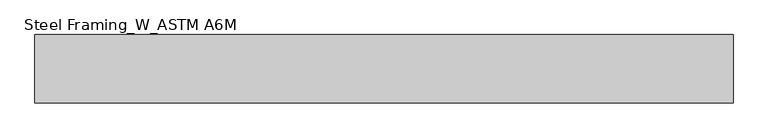
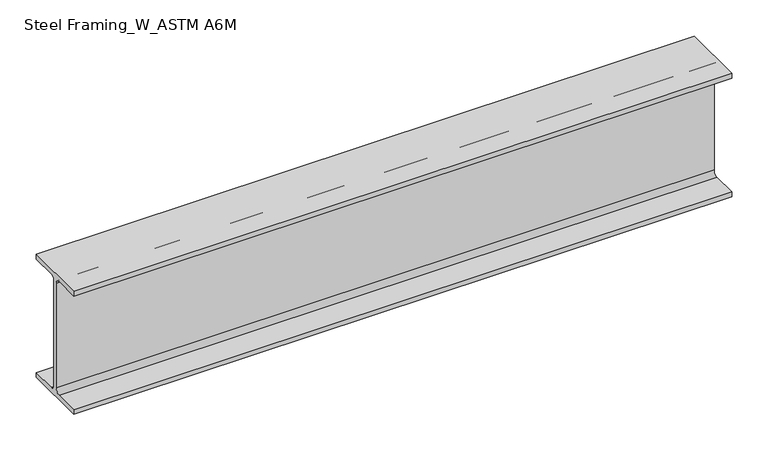
"""IFC4 building model written with IfcOpenShell, lengths in millimetres: beam geometry, Steel Framing_W_ASTM A6M : H_SB_AR_S02_W200x22.5_J1."""

from ifc_helpers import new_model, si_unit, point, frame, frame_2d, origin, place, context, project, spatial, polyline, circle_curve, trimmed, segment, composite_curve, outline, extrude, source, transform, mapped, element, save


def steel_framing_w_astm_a6m_f88b2983(model_context):
    return source(origin(), model_context, "Body", "SweptSolid", [
        extrude(outline(composite_curve([segment(polyline([(51.0, -95.0), (51.0, -103.0), (-51.0, -103.0), (-51.0, -95.0), (-10.71, -95.0)]), True, "CONTINUOUS"), segment(trimmed(circle_curve(frame_2d((-10.71, -87.4)), 7.6), [point((-10.71, -95.0))], [point((-3.11, -87.4))], True, "CARTESIAN"), True, "CONTINUOUS"), segment(polyline([(-3.11, -87.4), (-3.11, 87.4)]), True, "CONTINUOUS"), segment(trimmed(circle_curve(frame_2d((-10.71, 87.4)), 7.6), [point((-3.11, 87.4))], [point((-10.71, 95.0))], True, "CARTESIAN"), True, "CONTINUOUS"), segment(polyline([(-10.71, 95.0), (-51.0, 95.0), (-51.0, 103.0), (51.0, 103.0), (51.0, 95.0), (10.71, 95.0)]), True, "CONTINUOUS"), segment(trimmed(circle_curve(frame_2d((10.71, 87.4)), 7.6), [point((10.71, 95.0))], [point((3.11, 87.4))], True, "CARTESIAN"), True, "CONTINUOUS"), segment(polyline([(3.11, 87.4), (3.11, -87.4)]), True, "CONTINUOUS"), segment(trimmed(circle_curve(frame_2d((10.71, -87.4)), 7.6), [point((3.11, -87.4))], [point((10.71, -95.0))], True, "CARTESIAN"), True, "CONTINUOUS"), segment(polyline([(10.71, -95.0), (51.0, -95.0)]), True, "CONTINUOUS")], self_intersect=False)), frame((-520.3, 0.0, 0.0), z_axis=(1.0, 0.0, 0.0), x_axis=(0.0, 1.0, 0.0)), (0.0, 0.0, 1.0), 1040.6),
    ])


if __name__ == "__main__":
    model = new_model("IFC4")
    model_context = context("Model", 3, world=origin())
    ifc_project = project(units=[si_unit("LENGTHUNIT", "METRE", prefix="MILLI")], contexts=[model_context])
    site = spatial("IfcSite", under=ifc_project)
    building = spatial("IfcBuilding", under=site)
    placement = place(None, origin())
    steel_framing_w_astm_a6m_shape = steel_framing_w_astm_a6m_f88b2983(model_context)
    element("IfcBeam", 1, ObjectType="Steel Framing_W_ASTM A6M : H_SB_AR_S02_W200x22.5_J1", at=placement, inside=building, context=model_context, shape_type="MappedRepresentation", body=[
        mapped(steel_framing_w_astm_a6m_shape, transform((0.0, 0.0, 0.0), x_axis=(1.0, 0.0, 0.0), y_axis=(0.0, 1.0, 0.0), z_axis=(0.0, 0.0, 1.0))),
    ])
    save(model, "model.ifc")

# Revit data of these elements
# Type "Steel Framing_W_ASTM A6M : H_SB_AR_S02_W200x22.5_J1"
#   Section Name Key = "W8x15"
#   Width = 10.2 cm
#   Web Thickness = 0.622 cm
#   Web Fillet = 0.76 cm
#   Warping Constant = 13900.0 cm⁶
#   Torsional Moment of Inertia = 5.70 cm⁴
#   Section Area = 28.6 cm²
#   Plastic Modulus weak axis = 43.8 cm³
#   Plastic Modulus strong axis = 223.0 cm³
#   Perimeter = 0.795 m²/m
#   Nominal Weight = 22.50 kgf/m
#   Moment of Inertia weak axis = 142.00 cm⁴
#   Moment of Inertia strong axis = 2000.00 cm⁴
#   Height = 20.6 cm
#   Flange Thickness = 0.8 cm
#   Elastic Modulus weak axis = 27.9 cm³
#   Elastic Modulus strong axis = 193.0 cm³
#   Centroid Vertical = 10.3 cm
#   Centroid Horizontal = 5.1 cm
#   Length [instance default] = 1500 mm
#   Structural Material [instance default] = Steel, 45-345
#   Bolt Spacing = 0
#   Assembly Code = ""
# Element 1 (IfcBeam, "Steel Framing_W_ASTM A6M : H_SB_AR_S02_W200x22.5_J1")
#   Structural Material = Steel ASTM A36
#   Materials on its faces: "Steel ASTM A36"
# Materials
#   "Steel, 45-345": class "Metal", colour RGB 189 187 185, transparency 0, Description = "Steel 345 MPa", Cost = 0
#   "Steel ASTM A36": class "Metal", colour RGB 199 199 199, transparency 0, Description = "Structural steel, ASTM A36 Grade B, mill finish", Cost = 0
